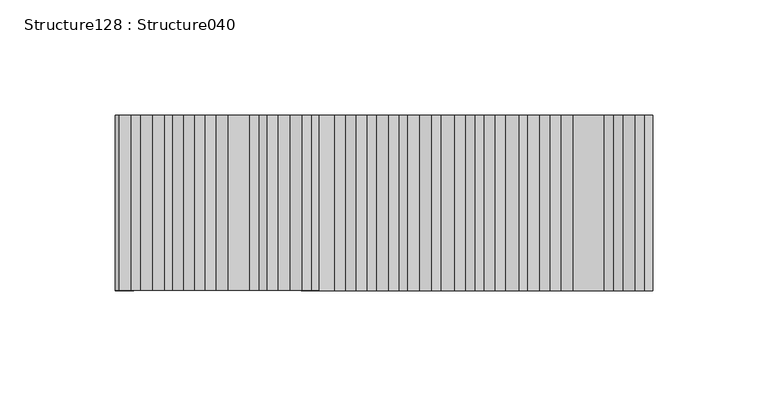
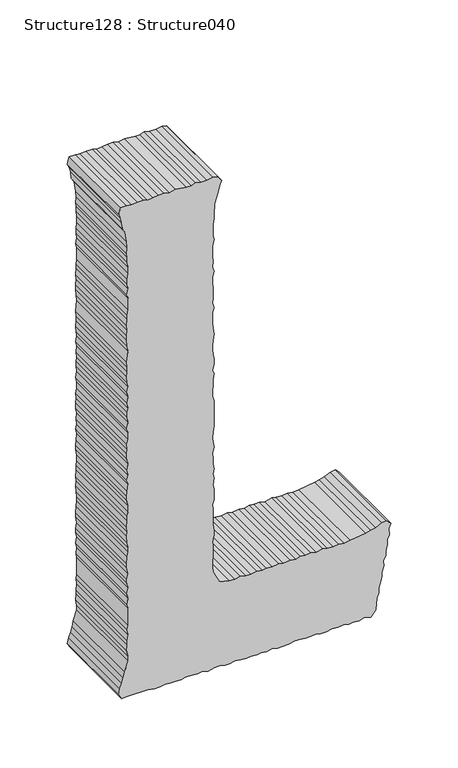
"""IFC4 building model written with IfcOpenShell, lengths in millimetres: proxy geometry, Structure128 : Structure040."""

from ifc_helpers import new_model, si_unit, frame, origin, place, context, project, spatial, polyline, outline, extrude, source, transform, mapped, element, save


def structure128_structure040_cb21a638(model_context):
    return source(origin(), model_context, "Body", "SweptSolid", [
        extrude(outline(polyline([(3629.5984101, -42569.665359), (3633.0980525, -42573.1874659), (3632.5155811, -42577.2647659), (3630.1824862, -42582.5695884), (3628.998288, -42586.648493), (3627.8397636, -42590.770722), (3626.0554434, -42604.2317491), (3625.472972, -42609.5141071), (3626.0554434, -42614.2155982), (3625.472972, -42618.8962296), (3626.0554434, -42624.1561231), (3626.6571701, -42627.6766254), (3625.472972, -42633.5382456), (3626.6571701, -42638.2172723), (3626.0554434, -42642.9203681), (3626.6571701, -42646.9992727), (3625.472972, -42651.1215016), (3626.0554434, -42655.802133), (3625.472972, -42661.6637532), (3626.6571701, -42665.7635177), (3625.472972, -42671.0234112), (3626.0554434, -42676.3057692), (3625.472972, -42679.8262715), (3626.0554434, -42684.5069028), (3625.472972, -42689.7651917), (3625.472972, -42693.8890253), (3626.6571701, -42698.5696566), (3625.472972, -42703.2711478), (3626.0554434, -42707.9517791), (3627.8397636, -42716.7321749), (3631.3410106, -42718.492426), (3638.9580681, -42722.0145329), (3643.0578326, -42722.5937951), (3648.9258713, -42722.5937951), (3652.9999621, -42722.0145329), (3662.9854159, -42722.0145329), (3666.5027089, -42722.5937951), (3672.3691429, -42721.4128062), (3676.4432338, -42721.4128062), (3681.7271964, -42722.0145329), (3695.786741, -42722.0145329), (3700.4705815, -42722.5937951), (3704.0135482, -42721.4128062), (3713.3555556, -42721.4128062), (3718.0554422, -42722.0145329), (3723.9154578, -42721.4128062), (3728.0152223, -42722.0145329), (3732.1149867, -42721.4128062), (3736.7988273, -42722.0145329), (3742.0747668, -42722.0145329), (3746.7586074, -42722.5937951), (3752.04257, -42721.4128062), (3756.7440611, -42722.0145329), (3760.2437036, -42722.5937951), (3766.1021146, -42722.0145329), (3770.8036057, -42721.4128062), (3793.6451507, -42721.4128062), (3798.3305959, -42722.5937951), (3803.0064134, -42722.5937951), (3808.290376, -42722.0145329), (3812.9726119, -42722.0145329), (3818.2309008, -42721.4128062), (3821.7722629, -42722.5937951), (3827.0321565, -42721.4128062), (3832.3161191, -42721.4128062), (3836.4174882, -42722.0145329), (3841.0900965, -42722.5937951), (3845.1914656, -42722.5937951), (3854.5751926, -42721.4128062), (3860.4432313, -42722.0145329), (3865.1190488, -42722.5937951), (3874.5043805, -42722.5937951), (3878.0024183, -42721.4128062), (3882.7039095, -42722.5937951), (3887.38775, -42722.0145329), (3896.763454, -42722.0145329), (3901.44569, -42722.5937951), (3906.7328618, -42722.5937951), (3911.4054701, -42721.4128062), (3915.5068392, -42722.5937951), (3920.7908018, -42722.0145329), (3925.4746423, -42722.5937951), (3934.2758979, -42722.5937951), (3940.1166583, -42721.4128062), (3943.6339514, -42722.0145329), (3953.5937315, -42722.0145329), (3958.8776941, -42721.4128062), (3962.9774586, -42721.4128062), (3972.3627903, -42720.833544), (3977.6194746, -42719.0941527), (3981.7208437, -42717.9131638), (3987.0048063, -42716.7321749), (3991.6806238, -42714.9719237), (3995.7803883, -42717.9131638), (3996.9645864, -42722.0145329), (3995.7803883, -42727.2728218), (3995.7803883, -42732.5551798), (3996.9645864, -42737.2358111), (3995.7803883, -42740.7563134), (3995.7803883, -42744.8576825), (3996.9645864, -42754.239805), (3995.7803883, -42759.4996985), (3996.9645864, -42764.2011897), (3996.9645864, -42768.881821), (3996.390138, -42773.5849168), (3995.7803883, -42778.2639435), (3996.9645864, -42781.7635859), (3996.9645864, -42787.0443393), (3996.390138, -42792.3266973), (3996.9645864, -42796.4056019), (3996.9645864, -42801.6863553), (3991.0788971, -42803.448211), (3987.5792547, -42801.6863553), (3982.8793681, -42800.5278308), (3977.0209571, -42799.9485686), (3972.9372387, -42797.5865908), (3964.1343784, -42796.4056019), (3958.8776941, -42795.8488041), (3953.5937315, -42796.4056019), (3950.0940891, -42795.8488041), (3945.4182716, -42795.8488041), (3940.718385, -42795.2470774), (3935.4328178, -42795.2470774), (3930.1745289, -42795.8488041), (3925.4746423, -42795.8488041), (3921.3748778, -42795.2470774), (3916.0909152, -42796.4056019), (3912.5896682, -42795.2470774), (3902.0201384, -42795.2470774), (3897.3475301, -42795.8488041), (3893.822214, -42795.8488041), (3887.9621984, -42796.4056019), (3883.8881076, -42795.8488041), (3879.1769888, -42796.4056019), (3875.0772243, -42796.4056019), (3869.2444869, -42795.8488041), (3864.5446004, -42795.2470774), (3855.1769193, -42796.4056019), (3850.4754282, -42795.8488041), (3846.3772683, -42795.8488041), (3841.6741725, -42796.4056019), (3836.4174882, -42795.8488041), (3832.3161191, -42795.2470774), (3827.6162325, -42796.4056019), (3823.5341187, -42795.2470774), (3817.6741031, -42795.8488041), (3812.9726119, -42795.2470774), (3809.4729695, -42795.8488041), (3804.7730829, -42795.8488041), (3800.0876378, -42795.2470774), (3794.8309535, -42796.4056019), (3790.7039107, -42795.2470774), (3784.8438951, -42795.2470774), (3780.7441306, -42796.4056019), (3776.0618947, -42795.8488041), (3771.9605256, -42796.4056019), (3767.2590344, -42796.4056019), (3762.5848215, -42795.2470774), (3756.7440611, -42795.8488041), (3752.04257, -42795.2470774), (3747.9428055, -42796.4056019), (3743.8414364, -42795.2470774), (3737.9750024, -42795.8488041), (3733.2991849, -42796.4056019), (3729.7738688, -42796.4056019), (3724.4979292, -42795.2470774), (3719.2316172, -42795.2470774), (3715.1302482, -42795.8488041), (3711.0304837, -42795.8488041), (3705.1720727, -42796.4056019), (3701.0723082, -42795.8488041), (3696.9709391, -42796.4056019), (3691.0868544, -42795.8488041), (3686.4030139, -42795.2470774), (3682.8857208, -42795.2470774), (3678.2018803, -42795.8488041), (3672.3691429, -42796.4056019), (3668.8261762, -42796.4056019), (3662.9854159, -42795.2470774), (3658.3015753, -42796.4056019), (3654.7842823, -42796.4056019), (3650.1004418, -42795.2470774), (3644.8245022, -42796.4056019), (3640.7167147, -42795.2470774), (3634.856699, -42795.8488041), (3631.3410106, -42795.2470774), (3616.0972679, -42795.2470774), (3612.0135494, -42795.8488041), (3607.3393366, -42795.2470774), (3602.0280957, -42795.8488041), (3598.5284533, -42795.8488041), (3593.2541183, -42796.4056019), (3587.9685511, -42795.2470774), (3583.8864372, -42795.2470774), (3575.0851816, -42798.1883175), (3569.8268927, -42799.3468419), (3565.1254015, -42800.5278308), (3561.025637, -42802.288082), (3555.7416744, -42803.448211), (3551.0658569, -42800.5278308), (3551.6675836, -42797.0073286), (3551.6675836, -42778.2639435), (3550.4833855, -42772.4023232), (3550.4833855, -42767.7008321), (3551.6675836, -42763.599463), (3551.0658569, -42759.4996985), (3551.0658569, -42754.239805), (3550.4833855, -42749.5367092), (3551.6675836, -42746.0386714), (3551.6675836, -42740.7563134), (3551.0658569, -42735.47556), (3551.6675836, -42731.9759176), (3550.4833855, -42726.716024), (3551.6675836, -42721.4128062), (3551.6675836, -42716.7321749), (3550.4833855, -42712.0290791), (3550.4833855, -42707.9517791), (3551.6675836, -42703.2711478), (3551.0658569, -42698.5696566), (3550.4833855, -42693.309763), (3551.0658569, -42689.7651917), (3550.4833855, -42684.5069028), (3551.0658569, -42681.0072604), (3550.4833855, -42676.3057692), (3551.6675836, -42671.0234112), (3550.4833855, -42666.9220421), (3550.4833855, -42657.5623841), (3551.6675836, -42651.7007639), (3551.6675836, -42646.9992727), (3551.0658569, -42642.9203681), (3551.0658569, -42638.2172723), (3551.6675836, -42633.5382456), (3550.4833855, -42630.0161387), (3550.4833855, -42624.7353853), (3551.6675836, -42620.054754), (3551.0658569, -42614.772396), (3551.6675836, -42610.0933693), (3550.4833855, -42605.412738), (3551.0658569, -42601.8922357), (3550.4833855, -42596.6323422), (3551.6675836, -42592.5085086), (3550.4833855, -42586.648493), (3555.7416744, -42582.5695884), (3561.025637, -42581.9678617), (3565.7094775, -42581.3885995), (3569.8268927, -42579.6283483), (3574.5107332, -42579.6283483), (3578.6104977, -42578.4457548), (3583.8864372, -42577.2647659), (3587.9685511, -42577.2647659), (3593.2541183, -42575.5269793), (3597.9540049, -42576.1287059), (3601.4536473, -42573.7667281), (3605.572667, -42573.7667281), (3611.4134274, -42572.5857392), (3616.0972679, -42572.5857392), (3619.6145609, -42570.8238835), (3625.472972, -42571.4256102), (3629.5984101, -42569.665359)])), frame((0.0, 247945.1599557, 0.0), z_axis=(0.0, 1.0, 0.0), x_axis=(0.0, 0.0, 1.0)), (0.0, 0.0, 1.0), 76.2),
    ])


if __name__ == "__main__":
    model = new_model("IFC4")
    model_context = context("Model", 3, world=origin())
    ifc_project = project(units=[si_unit("LENGTHUNIT", "METRE", prefix="MILLI")], contexts=[model_context])
    site = spatial("IfcSite", under=ifc_project)
    building = spatial("IfcBuilding", under=site)
    placement = place(None, origin())
    structure128_structure040_shape = structure128_structure040_cb21a638(model_context)
    element("IfcBuildingElementProxy", 1, Name="Structure128 : Structure040", ObjectType="Structure128 : Structure040", at=placement, inside=building, context=model_context, shape_type="MappedRepresentation", body=[
        mapped(structure128_structure040_shape, transform((0.0, 0.0, 0.0), x_axis=(1.0, 0.0, 0.0), y_axis=(0.0, 1.0, 0.0), z_axis=(0.0, 0.0, 1.0))),
    ])
    save(model, "model.ifc")

# Revit data of these elements
# Type "Structure128 : Structure040"
#   NameOverride = "Structure040"
# Element 1 (IfcBuildingElementProxy, "Structure128 : Structure040")
#   Materials on its faces: "BRUSHED ALUM. LETTERING"
# Materials
#   "BRUSHED ALUM. LETTERING": class "Unassigned", colour RGB 169 181 186, transparency 0, Cost = 0
